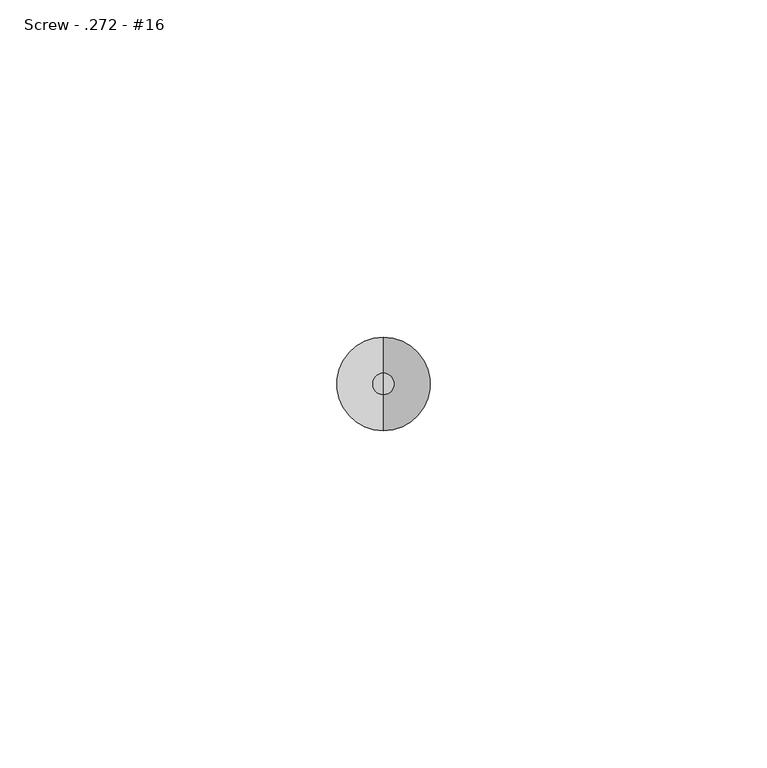
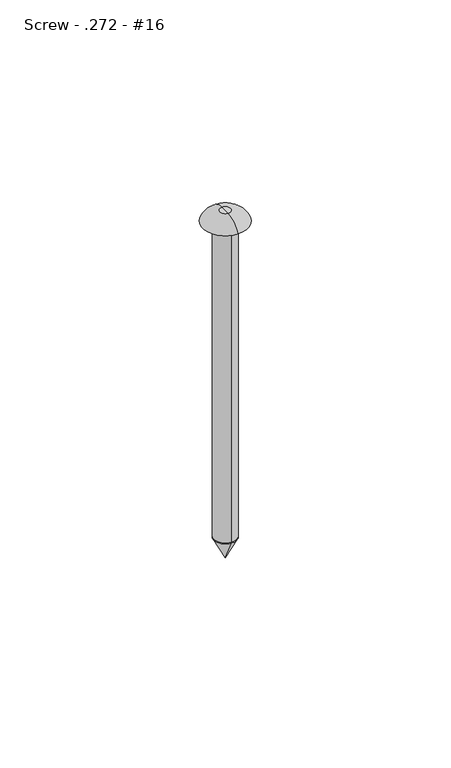
"""IFC4 building model written with IfcOpenShell, lengths in millimetres: fastener geometry, 060523 - W_P_C - Fastenings - Generic : Screw - .272 - #16."""

from ifc_helpers import new_model, si_unit, point, frame, origin, origin_2d, place, context, project, spatial, polyline, circle_curve, ellipse_curve, trimmed, segment, composite_curve, outline, extrude, source, transform, mapped, element, save
from ifc_brep_helpers import plane_surface, revolved_surface, advanced_brep


def screw_272_16_298fb2d3(model_context):
    return source(origin(), model_context, "Body", "SolidModel", [
        advanced_brep(
        [(0.0, -3.4544, -101.6), (0.0, 3.4544, -101.6), (0.0, 0.0, -101.6), (0.0, 0.0, -108.5088)],
        [
            (0, 1, circle_curve(frame((0.0, 0.0, -101.6), z_axis=(0.0, 0.0, 1.0), x_axis=(0.0, 1.0, 0.0)), 3.4544)),
            (1, 2),
            (2, 0),
            (1, 0, circle_curve(frame((0.0, 0.0, -101.6), z_axis=(0.0, 0.0, 1.0), x_axis=(0.0, 1.0, 0.0)), 3.4544)),
            (3, 1),
            (0, 3),
        ],
        [
            plane_surface(frame((0.0, 0.0, -101.6), z_axis=(0.0, 0.0, 1.0), x_axis=(0.0, 1.0, 0.0))),
            revolved_surface(polyline([(0.0, 3.4544, -101.6), (0.0, 0.0, -108.5088)]), (0.0, 0.0, -103.0840259), (0.0, 0.0, -1.0)),
        ],
        [
            (0, [[1, 2, 3]]),
            (0, [[4, -3, -2]]),
            (1, [[5, -1, 6]]),
            (1, [[-6, -4, -5]]),
        ],
    ),
        advanced_brep(
        [(0.0, 6.9088, 0.0), (0.0, -6.9088, 0.0), (0.0, 0.0, 0.0), (0.0, 0.0, 3.4544), (0.0, -1.5875, 3.4544), (0.0, 1.5875, 3.4544)],
        [
            (0, 1, circle_curve(frame((0.0, 0.0, 0.0), z_axis=(0.0, 0.0, -1.0), x_axis=(0.0, -1.0, 0.0)), 6.9088)),
            (1, 2),
            (2, 0),
            (1, 0, circle_curve(frame((0.0, 0.0, 0.0), z_axis=(0.0, 0.0, -1.0), x_axis=(0.0, -1.0, 0.0)), 6.9088)),
            (3, 4),
            (4, 5, circle_curve(frame((0.0, 0.0, 3.4544), z_axis=(0.0, 0.0, 1.0), x_axis=(0.0, -1.0, 0.0)), 1.5875)),
            (5, 3),
            (5, 4, circle_curve(frame((0.0, 0.0, 3.4544), z_axis=(0.0, 0.0, 1.0), x_axis=(0.0, -1.0, 0.0)), 1.5875)),
            (4, 1, circle_curve(frame((0.0, -1.5875, -2.3713748), z_axis=(1.0, 0.0, 0.0), x_axis=(0.0, -1.0, 0.0)), 5.8257748)),
            (0, 5, circle_curve(frame((0.0, 1.5875, -2.3713748), z_axis=(1.0, 0.0, 0.0), x_axis=(0.0, 1.0, 0.0)), 5.8257748)),
        ],
        [
            plane_surface(frame((0.0, 0.0, 0.0), z_axis=(0.0, 0.0, -1.0), x_axis=(0.0, -1.0, 0.0))),
            plane_surface(frame((0.0, 0.0, 3.4544), z_axis=(0.0, 0.0, 1.0), x_axis=(0.0, -1.0, 0.0))),
            revolved_surface(trimmed(ellipse_curve(frame((0.0, -1.5875, -2.3713748), z_axis=(-1.0, 0.0, 0.0), x_axis=(0.0, -1.0, 0.0)), 5.8257748, 5.8257748), [point((0.0, -6.9088, 0.0))], [point((0.0, -1.5875, 3.4544))], True, "CARTESIAN"), (0.0, 0.0, 1.4840259), (0.0, 0.0, 1.0)),
        ],
        [
            (0, [[1, 2, 3]]),
            (0, [[4, -3, -2]]),
            (1, [[5, 6, 7]]),
            (1, [[-7, 8, -5]]),
            (2, [[-6, 9, -1, 10]]),
            (2, [[-8, -10, -4, -9]]),
        ],
    ),
        extrude(outline(composite_curve([segment(trimmed(circle_curve(origin_2d(), 3.4544), [point((0.0, -3.4544))], [point((0.0, 3.4544))], False, "CARTESIAN"), True, "CONTINUOUS"), segment(trimmed(circle_curve(origin_2d(), 3.4544), [point((0.0, 3.4544))], [point((0.0, -3.4544))], False, "CARTESIAN"), True, "CONTINUOUS")], self_intersect=False)), frame((0.0, 0.0, -101.6), z_axis=(0.0, 0.0, 1.0), x_axis=(1.0, 0.0, 0.0)), (0.0, 0.0, 1.0), 101.6),
    ])


if __name__ == "__main__":
    model = new_model("IFC4")
    model_context = context("Model", 3, world=origin())
    ifc_project = project(units=[si_unit("LENGTHUNIT", "METRE", prefix="MILLI")], contexts=[model_context])
    site = spatial("IfcSite", under=ifc_project)
    building = spatial("IfcBuilding", under=site)
    placement = place(None, origin())
    screw_272_16_shape = screw_272_16_298fb2d3(model_context)
    element("IfcFastener", 1, ObjectType="060523 - W_P_C - Fastenings - Generic : Screw - .272 - #16", at=placement, inside=building, context=model_context, shape_type="MappedRepresentation", body=[
        mapped(screw_272_16_shape, transform((0.0, 0.0, 0.0), x_axis=(1.0, 0.0, 0.0), y_axis=(0.0, 1.0, 0.0), z_axis=(0.0, 0.0, 1.0))),
    ])
    save(model, "model.ifc")

# Revit data of these elements
# Type "060523 - W_P_C - Fastenings - Generic : Screw - .272 - #16"
#   Washer_Thickness = 0' - 0.00333"
#   Washer Radius = 0' - 0.146"
#   Washer Offset - Head = 0' - 0"
#   Washer Offset = 0' - 0"
#   Thickness_of_Substrate [instance default] = 0' - 1"
#   Side = 0' - 0 37/64"
#   Radius = 0' - 0.136"
#   Length [instance default] = 0' - 4"
#   Head Size = 0' - 1"
#   Head Radius = 0' - 0 1/2"
#   Head Height = 0' - 0.01"
#   Double Diameter = 0' - 0.544"
#   Diameter = 0' - 0.272"
#   Default Elevation = 4' - 0"
#   Washer_Nut_Visibility = no
#   Washer_Head_Visibility = no
#   Round_Head_Visibility = yes
#   Point Visibility = yes
#   Nut_Visibility = no
#   Hex_Head_Visiblilty = no
#   Washer Material = none
#   Bolt Material (Size) = AT SILL - FASTENER AT 24" O.C.
# Element 1 (IfcFastener, "060523 - W_P_C - Fastenings - Generic : Screw - .272 - #16")
#   Materials on its faces: "AT SILL - FASTENER AT 24\" O.C."
# Materials
#   "AT SILL - FASTENER AT 24\" O.C.": class "Generic", colour RGB 120 120 120, transparency 0, Cost = 0
